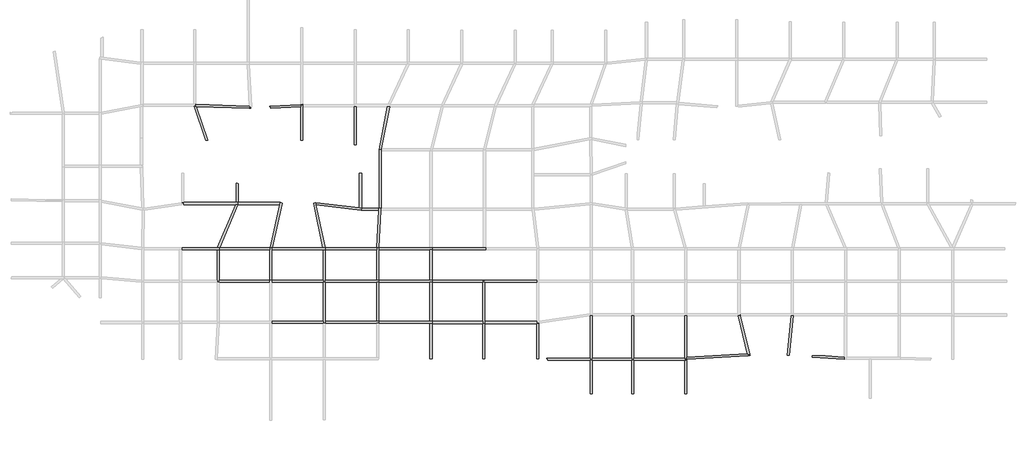
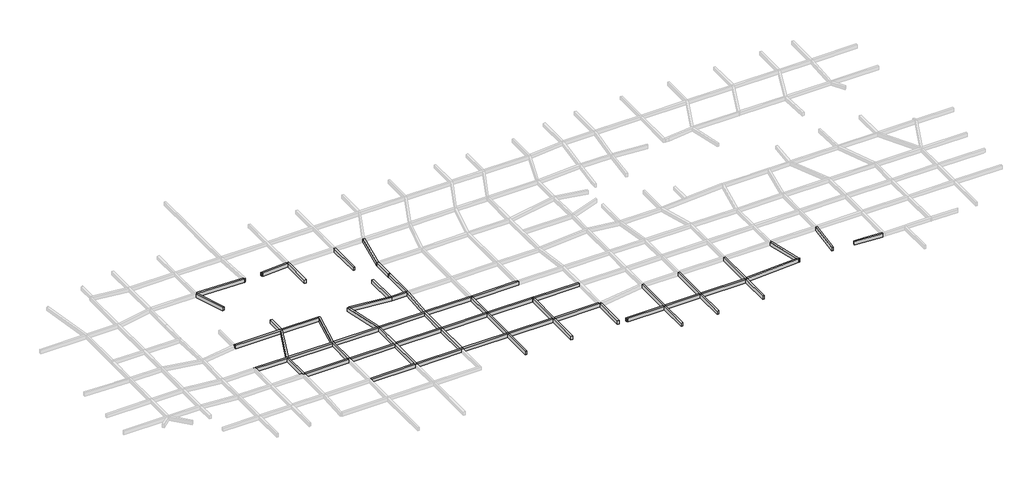
# One storey, part 4 of 15: 59 beams.
"""IFC4 building model written with IfcOpenShell, lengths in millimetres."""

from ifc_helpers import new_model, si_unit, frame, origin, place, context, project, spatial, polyline, outline, extrude, faceted_brep, element, save

model = new_model("IFC4")

# Units and contexts
model_context = context("Model", 3, world=origin())
ifc_project = project(units=[si_unit("LENGTHUNIT", "METRE", prefix="MILLI")], contexts=[model_context])

# Site, building, storey
site = spatial("IfcSite", under=ifc_project)
building = spatial("IfcBuilding", under=site)
storey = spatial("IfcBuildingStorey", under=building, Name="层高", Elevation=3300.0)

# Beams
placement = place(None, origin())
element("IfcBeam", 1, ObjectType="混凝土 - 矩形梁 : KL_beam", at=placement, inside=storey, context=model_context, shape_type="Brep", body=[
    faceted_brep([(169630.5037973, 63694.2273331, 3300.0), (169630.5037973, 63694.2273331, 2700.0), (169633.596084, 63790.1042703, 2700.0), (169633.596084, 63790.1042703, 3300.0), (169549.1301124, 63790.1042703, 2700.0), (169549.1301124, 63790.1042703, 3300.0), (169549.1301124, 63696.8518513, 2700.0), (169549.1301124, 63696.8518513, 3300.0)], [[[0, 1, 2, 3]], [[3, 2, 4, 5]], [[6, 7, 5, 4]], [[1, 0, 7, 6]], [[0, 3, 5, 7]], [[2, 1, 6, 4]]]),
    faceted_brep([(161497.8826169, 63956.5260367, 3300.0), (161497.8826169, 63956.5260367, 2700.0), (161712.9819644, 63949.5885096, 2700.0), (169429.1301124, 63700.722171, 2700.0), (169429.1301124, 63700.722171, 3300.0), (161712.9819644, 63949.5885096, 3300.0), (161650.300938, 63956.5260367, 3300.0), (161650.300938, 63956.5260367, 2700.0), (161650.300938, 64251.7661343, 3300.0), (161650.300938, 64251.7661343, 2700.0), (169429.1301124, 63790.1042703, 3300.0), (169429.1301124, 63910.1042703, 3300.0), (169481.9445066, 63910.1042703, 3300.0), (169477.2686164, 63999.3255706, 3300.0), (169477.2686164, 63999.3255706, 2700.0), (169481.9445066, 63910.1042703, 2700.0), (169429.1301124, 63910.1042703, 2700.0)], [[[0, 1, 2, 3, 4, 5]], [[6, 7, 1, 0]], [[7, 6, 8, 9]], [[6, 0, 5, 4, 10, 11, 12, 13, 8]], [[9, 8, 13, 14]], [[1, 7, 9, 14, 15, 16, 3, 2]], [[14, 13, 12, 15]], [[11, 16, 15, 12]], [[16, 11, 10, 4, 3]]]),
])
element("IfcBeam", 2, ObjectType="混凝土 - 矩形梁 : KL_beam", at=placement, inside=storey, context=model_context, shape_type="SweptSolid", body=[
    extrude(outline(polyline([(161393.3069779, 63956.5260367), (161497.8826169, 63956.5260367), (161712.9819644, 63949.5885096), (163398.0336281, 59055.8431382), (163080.7474238, 59055.8431382), (161393.3069779, 63956.5260367)])), frame((0.0, 0.0, 2700.0), z_axis=(0.0, 0.0, 1.0), x_axis=(1.0, 0.0, 0.0)), (0.0, 0.0, 1.0), 600.0),
])
element("IfcBeam", 3, ObjectType="混凝土 - 矩形梁 : KL_beam", at=placement, inside=storey, context=model_context, shape_type="Brep", body=[
    faceted_brep([(159257.4396146, 43339.5188273, 3300.0), (159549.7804968, 43339.3698411, 3300.0), (159549.7804968, 43042.2492414, 3300.0), (164749.7804968, 43042.2492414, 3300.0), (165049.7804968, 43042.2492414, 3300.0), (165049.7804968, 43342.2492414, 3300.0), (164801.5143118, 43342.2492414, 3300.0), (159257.5827095, 43342.2492414, 3300.0), (159549.7804968, 43042.2492414, 2700.0), (164749.7804968, 43042.2492414, 2700.0), (165049.7804968, 43042.2492414, 2700.0), (159549.7804968, 43339.3698411, 2700.0), (159257.4396146, 43339.5188273, 2700.0), (159257.5827095, 43342.2492414, 2700.0), (164801.5143118, 43342.2492414, 2700.0), (165049.7804968, 43342.2492414, 2700.0)], [[[0, 1, 2, 3, 4, 5, 6, 7]], [[2, 8, 9, 10, 4, 3]], [[11, 12, 13, 14, 15, 10, 9, 8]], [[5, 15, 14, 13, 7, 6]], [[11, 1, 0, 12]], [[1, 11, 8, 2]], [[5, 4, 10, 15]], [[7, 13, 12, 0]]]),
])
element("IfcBeam", 4, ObjectType="混凝土 - 矩形梁 : KL_beam", at=placement, inside=storey, context=model_context, shape_type="Brep", body=[
    faceted_brep([(164749.7804968, 38266.5295438, 3300.0), (165049.7804968, 38266.5295438, 3300.0), (165049.7804968, 38566.5295438, 3300.0), (165049.7804968, 43042.2492414, 3300.0), (164749.7804968, 43042.2492414, 3300.0), (164749.7804968, 38566.5295438, 3300.0), (164749.7804968, 38266.5295438, 2700.0), (164749.7804968, 43042.2492414, 2700.0), (164749.7804968, 38566.5295438, 2700.0), (165049.7804968, 38266.5295438, 2700.0), (165049.7804968, 43042.2492414, 2700.0), (165049.7804968, 38566.5295438, 2700.0)], [[[0, 1, 2, 3, 4, 5]], [[6, 0, 5, 4, 7, 8]], [[9, 6, 8, 7, 10, 11]], [[1, 9, 11, 10, 3, 2]], [[4, 3, 10, 7]], [[1, 0, 6, 9]]]),
])
element("IfcBeam", 5, ObjectType="混凝土 - 矩形梁 : KL_beam", at=placement, inside=storey, context=model_context, shape_type="SweptSolid", body=[
    extrude(outline(polyline([(165049.7804968, 38266.5295438), (165049.7804968, 38566.5295438), (172449.7804968, 38566.5295438), (172449.7804968, 38266.5295438), (165049.7804968, 38266.5295438)])), frame((0.0, 0.0, 2700.0), z_axis=(0.0, 0.0, 1.0), x_axis=(1.0, 0.0, 0.0)), (0.0, 0.0, 1.0), 600.0),
])
element("IfcBeam", 6, ObjectType="混凝土 - 矩形梁 : KL_beam", at=placement, inside=storey, context=model_context, shape_type="Brep", body=[
    faceted_brep([(172749.7804968, 43342.2492414, 3300.0), (172481.1122271, 43342.2492414, 3300.0), (172449.7804968, 43342.2492414, 3300.0), (172449.7804968, 43042.2492414, 3300.0), (172449.7804968, 38566.5295438, 3300.0), (172749.7804968, 38566.5295438, 3300.0), (172749.7804968, 43042.2492414, 3300.0), (172449.7804968, 43342.2492414, 2700.0), (172449.7804968, 43042.2492414, 2700.0), (172449.7804968, 38566.5295438, 2700.0), (172481.1122271, 43342.2492414, 2700.0), (172749.7804968, 43342.2492414, 2700.0), (172749.7804968, 43042.2492414, 2700.0), (172749.7804968, 38566.5295438, 2700.0)], [[[0, 1, 2, 3, 4, 5, 6]], [[2, 7, 8, 9, 4, 3]], [[7, 10, 11, 12, 13, 9, 8]], [[11, 0, 6, 5, 13, 12]], [[5, 4, 9, 13]], [[2, 1, 0, 11, 10, 7]]]),
])
element("IfcBeam", 7, ObjectType="混凝土 - 矩形梁 : KL_beam", at=placement, inside=storey, context=model_context, shape_type="Brep", body=[
    faceted_brep([(165049.7804968, 43342.2492414, 3300.0), (165049.7804968, 43042.2492414, 3300.0), (172449.7804968, 43042.2492414, 3300.0), (172449.7804968, 43342.2492414, 3300.0), (165127.2075965, 43342.2492414, 3300.0), (165049.7804968, 43042.2492414, 2700.0), (172449.7804968, 43042.2492414, 2700.0), (165049.7804968, 43342.2492414, 2700.0), (165127.2075965, 43342.2492414, 2700.0), (172449.7804968, 43342.2492414, 2700.0)], [[[0, 1, 2, 3, 4]], [[1, 5, 6, 2]], [[5, 7, 8, 9, 6]], [[7, 0, 4, 3, 9, 8]], [[1, 0, 7, 5]], [[3, 2, 6, 9]]]),
])
element("IfcBeam", 8, ObjectType="混凝土 - 矩形梁 : KL_beam", at=placement, inside=storey, context=model_context, shape_type="Brep", body=[
    faceted_brep([(180549.7804968, 43042.2492414, 3300.0), (180549.7804968, 43342.2492414, 3300.0), (180520.652311, 43342.2492414, 3300.0), (180213.9501326, 43342.2492414, 3300.0), (172789.0034594, 43342.2492414, 3300.0), (172749.7804968, 43342.2492414, 3300.0), (172749.7804968, 43042.2492414, 3300.0), (180249.7804968, 43042.2492414, 3300.0), (180549.7804968, 43042.2492414, 2700.0), (172749.7804968, 43042.2492414, 2700.0), (180249.7804968, 43042.2492414, 2700.0), (180549.7804968, 43342.2492414, 2700.0), (172749.7804968, 43342.2492414, 2700.0), (172789.0034594, 43342.2492414, 2700.0), (180213.9501326, 43342.2492414, 2700.0), (180520.652311, 43342.2492414, 2700.0)], [[[0, 1, 2, 3, 4, 5, 6, 7]], [[8, 0, 7, 6, 9, 10]], [[11, 8, 10, 9, 12, 13, 14, 15]], [[1, 11, 15, 14, 13, 12, 5, 4, 3, 2]], [[6, 5, 12, 9]], [[1, 0, 8, 11]]]),
])
element("IfcBeam", 9, ObjectType="混凝土 - 矩形梁 : KL_beam", at=placement, inside=storey, context=model_context, shape_type="Brep", body=[
    faceted_brep([(180249.7804968, 38266.5295438, 3300.0), (180549.7804968, 38266.5295438, 3300.0), (180549.7804968, 38566.5295438, 3300.0), (180549.7804968, 43042.2492414, 3300.0), (180249.7804968, 43042.2492414, 3300.0), (180249.7804968, 38566.5295438, 3300.0), (180549.7804968, 38266.5295438, 2700.0), (180549.7804968, 38566.5295438, 2700.0), (180549.7804968, 43042.2492414, 2700.0), (180249.7804968, 38266.5295438, 2700.0), (180249.7804968, 38566.5295438, 2700.0), (180249.7804968, 43042.2492414, 2700.0)], [[[0, 1, 2, 3, 4, 5]], [[1, 6, 7, 8, 3, 2]], [[6, 9, 10, 11, 8, 7]], [[9, 0, 5, 4, 11, 10]], [[4, 3, 8, 11]], [[1, 0, 9, 6]]]),
])
element("IfcBeam", 10, ObjectType="混凝土 - 矩形梁 : KL_beam", at=placement, inside=storey, context=model_context, shape_type="SweptSolid", body=[
    extrude(outline(polyline([(172749.7804968, 38266.5295438), (172749.7804968, 38566.5295438), (180249.7804968, 38566.5295438), (180249.7804968, 38266.5295438), (172749.7804968, 38266.5295438)])), frame((0.0, 0.0, 2700.0), z_axis=(0.0, 0.0, 1.0), x_axis=(1.0, 0.0, 0.0)), (0.0, 0.0, 1.0), 600.0),
])
element("IfcBeam", 11, ObjectType="混凝土 - 矩形梁 : KL_beam", at=placement, inside=storey, context=model_context, shape_type="Brep", body=[
    faceted_brep([(180249.7804968, 32266.5295438, 3300.0), (180549.7804968, 32266.5295438, 3300.0), (180549.7804968, 32566.5295438, 3300.0), (180549.7804968, 38266.5295438, 3300.0), (180249.7804968, 38266.5295438, 3300.0), (180249.7804968, 32566.5295438, 3300.0), (180249.7804968, 32266.5295438, 2700.0), (180249.7804968, 38266.5295438, 2700.0), (180249.7804968, 32566.5295438, 2700.0), (180549.7804968, 32266.5295438, 2700.0), (180549.7804968, 38266.5295438, 2700.0), (180549.7804968, 32566.5295438, 2700.0)], [[[0, 1, 2, 3, 4, 5]], [[6, 0, 5, 4, 7, 8]], [[9, 6, 8, 7, 10, 11]], [[1, 9, 11, 10, 3, 2]], [[4, 3, 10, 7]], [[1, 0, 6, 9]]]),
])
element("IfcBeam", 12, ObjectType="混凝土 - 矩形梁 : KL_beam", at=placement, inside=storey, context=model_context, shape_type="SweptSolid", body=[
    extrude(outline(polyline([(172749.7804968, 32266.5295438), (172749.7804968, 32566.5295438), (180249.7804968, 32566.5295438), (180249.7804968, 32266.5295438), (172749.7804968, 32266.5295438)])), frame((0.0, 0.0, 2700.0), z_axis=(0.0, 0.0, 1.0), x_axis=(1.0, 0.0, 0.0)), (0.0, 0.0, 1.0), 600.0),
])
element("IfcBeam", 13, ObjectType="混凝土 - 矩形梁 : KL_beam", at=placement, inside=storey, context=model_context, shape_type="Brep", body=[
    faceted_brep([(188349.7804968, 32266.5295438, 3300.0), (188349.7804968, 32566.5295438, 3300.0), (188049.7804968, 32566.5295438, 3300.0), (180549.7804968, 32566.5295438, 3300.0), (180549.7804968, 32266.5295438, 3300.0), (188049.7804968, 32266.5295438, 3300.0), (188349.7804968, 32266.5295438, 2700.0), (180549.7804968, 32266.5295438, 2700.0), (188049.7804968, 32266.5295438, 2700.0), (188349.7804968, 32566.5295438, 2700.0), (180549.7804968, 32566.5295438, 2700.0), (188049.7804968, 32566.5295438, 2700.0)], [[[0, 1, 2, 3, 4, 5]], [[6, 0, 5, 4, 7, 8]], [[9, 6, 8, 7, 10, 11]], [[1, 9, 11, 10, 3, 2]], [[4, 3, 10, 7]], [[1, 0, 6, 9]]]),
])
element("IfcBeam", 14, ObjectType="混凝土 - 矩形梁 : KL_beam", at=placement, inside=storey, context=model_context, shape_type="Brep", body=[
    faceted_brep([(188349.7804968, 38266.5295438, 3300.0), (188349.7804968, 38566.5295438, 3300.0), (188049.7804968, 38566.5295438, 3300.0), (180549.7804968, 38566.5295438, 3300.0), (180549.7804968, 38266.5295438, 3300.0), (188049.7804968, 38266.5295438, 3300.0), (188349.7804968, 38266.5295438, 2700.0), (180549.7804968, 38266.5295438, 2700.0), (188049.7804968, 38266.5295438, 2700.0), (188349.7804968, 38566.5295438, 2700.0), (180549.7804968, 38566.5295438, 2700.0), (188049.7804968, 38566.5295438, 2700.0)], [[[0, 1, 2, 3, 4, 5]], [[6, 0, 5, 4, 7, 8]], [[9, 6, 8, 7, 10, 11]], [[1, 9, 11, 10, 3, 2]], [[4, 3, 10, 7]], [[1, 0, 6, 9]]]),
])
element("IfcBeam", 15, ObjectType="混凝土 - 矩形梁 : KL_beam", at=placement, inside=storey, context=model_context, shape_type="SweptSolid", body=[
    extrude(outline(polyline([(188349.7804968, 32566.5295438), (188049.7804968, 32566.5295438), (188049.7804968, 38266.5295438), (188349.7804968, 38266.5295438), (188349.7804968, 32566.5295438)])), frame((0.0, 0.0, 2700.0), z_axis=(0.0, 0.0, 1.0), x_axis=(1.0, 0.0, 0.0)), (0.0, 0.0, 1.0), 600.0),
])
element("IfcBeam", 16, ObjectType="混凝土 - 矩形梁 : KL_beam", at=placement, inside=storey, context=model_context, shape_type="Brep", body=[
    faceted_brep([(188349.7804968, 43342.2492414, 3300.0), (188057.5827095, 43342.2492414, 3300.0), (188049.7804968, 43342.2492414, 3300.0), (188049.7804968, 43042.2492414, 3300.0), (188049.7804968, 38566.5295438, 3300.0), (188349.7804968, 38566.5295438, 3300.0), (188349.7804968, 43042.2492414, 3300.0), (188049.7804968, 43342.2492414, 2700.0), (188049.7804968, 43042.2492414, 2700.0), (188049.7804968, 38566.5295438, 2700.0), (188057.5827095, 43342.2492414, 2700.0), (188349.7804968, 43342.2492414, 2700.0), (188349.7804968, 43042.2492414, 2700.0), (188349.7804968, 38566.5295438, 2700.0)], [[[0, 1, 2, 3, 4, 5, 6]], [[2, 7, 8, 9, 4, 3]], [[7, 10, 11, 12, 13, 9, 8]], [[11, 0, 6, 5, 13, 12]], [[5, 4, 9, 13]], [[2, 1, 0, 11, 10, 7]]]),
])
element("IfcBeam", 17, ObjectType="混凝土 - 矩形梁 : KL_beam", at=placement, inside=storey, context=model_context, shape_type="SweptSolid", body=[
    extrude(outline(polyline([(180549.7804968, 43042.2492414), (180549.7804968, 43342.2492414), (188049.7804968, 43342.2492414), (188049.7804968, 43042.2492414), (180549.7804968, 43042.2492414)])), frame((0.0, 0.0, 2700.0), z_axis=(0.0, 0.0, 1.0), x_axis=(1.0, 0.0, 0.0)), (0.0, 0.0, 1.0), 600.0),
])
element("IfcBeam", 18, ObjectType="混凝土 - 矩形梁 : KL_beam", at=placement, inside=storey, context=model_context, shape_type="Brep", body=[
    faceted_brep([(196149.7804968, 43042.2492414, 3300.0), (196149.7804968, 43342.2492414, 3300.0), (195849.7804968, 43342.2492414, 3300.0), (188357.9944133, 43342.2492414, 3300.0), (188349.7804968, 43342.2492414, 3300.0), (188349.7804968, 43042.2492414, 3300.0), (195849.7804968, 43042.2492414, 3300.0), (196149.7804968, 43042.2492414, 2700.0), (188349.7804968, 43042.2492414, 2700.0), (195849.7804968, 43042.2492414, 2700.0), (196149.7804968, 43342.2492414, 2700.0), (188349.7804968, 43342.2492414, 2700.0), (188357.9944133, 43342.2492414, 2700.0), (195849.7804968, 43342.2492414, 2700.0)], [[[0, 1, 2, 3, 4, 5, 6]], [[7, 0, 6, 5, 8, 9]], [[10, 7, 9, 8, 11, 12, 13]], [[1, 10, 13, 12, 11, 4, 3, 2]], [[5, 4, 11, 8]], [[1, 0, 7, 10]]]),
])
element("IfcBeam", 19, ObjectType="混凝土 - 矩形梁 : KL_beam", at=placement, inside=storey, context=model_context, shape_type="Brep", body=[
    faceted_brep([(196149.7804968, 38266.5295438, 3300.0), (196149.7804968, 38566.5295438, 3300.0), (195849.7804968, 38566.5295438, 3300.0), (188349.7804968, 38566.5295438, 3300.0), (188349.7804968, 38266.5295438, 3300.0), (195849.7804968, 38266.5295438, 3300.0), (196149.7804968, 38266.5295438, 2700.0), (188349.7804968, 38266.5295438, 2700.0), (195849.7804968, 38266.5295438, 2700.0), (196149.7804968, 38566.5295438, 2700.0), (188349.7804968, 38566.5295438, 2700.0), (195849.7804968, 38566.5295438, 2700.0)], [[[0, 1, 2, 3, 4, 5]], [[6, 0, 5, 4, 7, 8]], [[9, 6, 8, 7, 10, 11]], [[1, 9, 11, 10, 3, 2]], [[4, 3, 10, 7]], [[1, 0, 6, 9]]]),
])
element("IfcBeam", 20, ObjectType="混凝土 - 矩形梁 : KL_beam", at=placement, inside=storey, context=model_context, shape_type="Brep", body=[
    faceted_brep([(196149.7804968, 32266.5295438, 3300.0), (196149.7804968, 32542.26105, 3300.0), (196149.7804968, 32566.5295438, 3300.0), (195849.7804968, 32566.5295438, 3300.0), (188349.7804968, 32566.5295438, 3300.0), (188349.7804968, 32266.5295438, 3300.0), (195849.7804968, 32266.5295438, 3300.0), (196149.7804968, 32266.5295438, 2700.0), (188349.7804968, 32266.5295438, 2700.0), (195849.7804968, 32266.5295438, 2700.0), (196149.7804968, 32566.5295438, 2700.0), (196149.7804968, 32542.26105, 2700.0), (188349.7804968, 32566.5295438, 2700.0), (195849.7804968, 32566.5295438, 2700.0)], [[[0, 1, 2, 3, 4, 5, 6]], [[7, 0, 6, 5, 8, 9]], [[10, 11, 7, 9, 8, 12, 13]], [[2, 10, 13, 12, 4, 3]], [[5, 4, 12, 8]], [[2, 1, 0, 7, 11, 10]]]),
])
element("IfcBeam", 21, ObjectType="混凝土 - 矩形梁 : KL_beam", at=placement, inside=storey, context=model_context, shape_type="SweptSolid", body=[
    extrude(outline(polyline([(195849.7804968, 38266.5295438), (196149.7804968, 38266.5295438), (196149.7804968, 32566.5295438), (195849.7804968, 32566.5295438), (195849.7804968, 38266.5295438)])), frame((0.0, 0.0, 2700.0), z_axis=(0.0, 0.0, 1.0), x_axis=(1.0, 0.0, 0.0)), (0.0, 0.0, 1.0), 600.0),
])
element("IfcBeam", 22, ObjectType="混凝土 - 矩形梁 : KL_beam", at=placement, inside=storey, context=model_context, shape_type="SweptSolid", body=[
    extrude(outline(polyline([(195849.7804968, 43042.2492414), (196149.7804968, 43042.2492414), (196149.7804968, 38566.5295438), (195849.7804968, 38566.5295438), (195849.7804968, 43042.2492414)])), frame((0.0, 0.0, 2700.0), z_axis=(0.0, 0.0, 1.0), x_axis=(1.0, 0.0, 0.0)), (0.0, 0.0, 1.0), 600.0),
])
element("IfcBeam", 23, ObjectType="混凝土 - 矩形梁 : KL_beam", at=placement, inside=storey, context=model_context, shape_type="Brep", body=[
    faceted_brep([(174002.1069516, 49930.4011957, 3300.0), (173932.8464943, 49630.4011957, 3300.0), (172481.1122271, 43342.2492414, 3300.0), (172749.7804968, 43342.2492414, 3300.0), (172789.0034594, 43342.2492414, 3300.0), (174275.6873874, 49781.7848082, 3300.0), (174260.3009401, 49781.7848082, 3300.0), (174140.3009401, 49781.7848082, 3300.0), (174140.3009401, 49898.4965996, 3300.0), (172789.0034594, 43342.2492414, 2700.0), (174275.6873874, 49781.7848082, 2700.0), (172481.1122271, 43342.2492414, 2700.0), (173932.8464943, 49630.4011957, 2700.0), (174002.1069516, 49930.4011957, 2700.0), (174140.3009401, 49898.4965996, 2700.0), (174140.3009401, 49781.7848082, 2700.0), (172749.7804968, 43342.2492414, 2700.0)], [[[0, 1, 2, 3, 4, 5, 6, 7, 8]], [[4, 9, 10, 5]], [[11, 12, 13, 14, 15, 10, 9, 16]], [[2, 1, 0, 13, 12, 11]], [[2, 11, 16, 9, 4, 3]], [[13, 0, 8, 14]], [[7, 15, 14, 8]], [[15, 7, 6, 5, 10]]]),
])
element("IfcBeam", 24, ObjectType="混凝土 - 矩形梁 : KL_beam", at=placement, inside=storey, context=model_context, shape_type="Brep", body=[
    faceted_brep([(180520.652311, 43342.2492414, 3300.0), (179195.182726, 49578.0933603, 3300.0), (179129.3076558, 49888.0111993, 3300.0), (179060.3009401, 49873.3433691, 3300.0), (179060.3009401, 49781.7848082, 3300.0), (178845.1845937, 49781.7848082, 3300.0), (180213.9501326, 43342.2492414, 3300.0), (180249.7804968, 43342.2492414, 3300.0), (180520.652311, 43342.2492414, 2700.0), (179195.182726, 49578.0933603, 2700.0), (179129.3076558, 49888.0111993, 2700.0), (180249.7804968, 43342.2492414, 2700.0), (180213.9501326, 43342.2492414, 2700.0), (178845.1845937, 49781.7848082, 2700.0), (179060.3009401, 49781.7848082, 2700.0), (179060.3009401, 49873.3433691, 2700.0)], [[[0, 1, 2, 3, 4, 5, 6, 7]], [[2, 1, 0, 8, 9, 10]], [[10, 9, 8, 11, 12, 13, 14, 15]], [[12, 6, 5, 13]], [[8, 0, 7, 6, 12, 11]], [[2, 10, 15, 3]], [[4, 14, 13, 5]], [[14, 4, 3, 15]]]),
])
element("IfcBeam", 25, ObjectType="混凝土 - 矩形梁 : KL_beam", at=placement, inside=storey, context=model_context, shape_type="Brep", body=[
    faceted_brep([(167784.8242353, 49930.4011957, 3300.0), (167535.3734044, 49930.4011957, 3300.0), (159895.197808, 49930.4011957, 3300.0), (159602.853123, 49930.4011957, 3300.0), (159601.8562875, 49911.380442, 3300.0), (159901.445148, 49895.6796551, 3300.0), (159888.5393285, 49649.4219495, 3300.0), (159887.542493, 49630.4011957, 3300.0), (167459.1309506, 49630.4011957, 3300.0), (167784.8242353, 49630.4011957, 3300.0), (159887.542493, 49630.4011957, 2700.0), (167459.1309506, 49630.4011957, 2700.0), (167784.8242353, 49630.4011957, 2700.0), (159602.853123, 49930.4011957, 2700.0), (159895.197808, 49930.4011957, 2700.0), (167535.3734044, 49930.4011957, 2700.0), (167784.8242353, 49930.4011957, 2700.0), (159888.5393285, 49649.4219495, 2700.0), (159901.445148, 49895.6796551, 2700.0), (159601.8562875, 49911.380442, 2700.0)], [[[0, 1, 2, 3, 4, 5, 6, 7, 8, 9]], [[9, 8, 7, 10, 11, 12]], [[13, 14, 15, 16, 12, 11, 10, 17, 18, 19]], [[3, 2, 1, 0, 16, 15, 14, 13]], [[19, 4, 3, 13]], [[5, 18, 17, 10, 7, 6]], [[18, 5, 4, 19]], [[0, 9, 12, 16]]]),
])
element("IfcBeam", 26, ObjectType="混凝土 - 矩形梁 : KL_beam", at=placement, inside=storey, context=model_context, shape_type="Brep", body=[
    faceted_brep([(173932.8464943, 49630.4011957, 3300.0), (174002.1069516, 49930.4011957, 3300.0), (167835.3734044, 49930.4011957, 3300.0), (167784.8242353, 49930.4011957, 3300.0), (167784.8242353, 49630.4011957, 3300.0), (173932.8464943, 49630.4011957, 2700.0), (167784.8242353, 49630.4011957, 2700.0), (174002.1069516, 49930.4011957, 2700.0), (167784.8242353, 49930.4011957, 2700.0), (167835.3734044, 49930.4011957, 2700.0)], [[[0, 1, 2, 3, 4]], [[5, 0, 4, 6]], [[7, 5, 6, 8, 9]], [[1, 7, 9, 8, 3, 2]], [[1, 0, 5, 7]], [[4, 3, 8, 6]]]),
])
element("IfcBeam", 27, ObjectType="混凝土 - 矩形梁 : KL_beam", at=placement, inside=storey, context=model_context, shape_type="Brep", body=[
    faceted_brep([(165127.2075965, 43342.2492414, 3300.0), (167784.8242353, 49630.4011957, 3300.0), (167459.1309506, 49630.4011957, 3300.0), (164801.5143118, 43342.2492414, 3300.0), (165049.7804968, 43342.2492414, 3300.0), (164801.5143118, 43342.2492414, 2700.0), (167459.1309506, 49630.4011957, 2700.0), (167784.8242353, 49630.4011957, 2700.0), (165127.2075965, 43342.2492414, 2700.0), (165049.7804968, 43342.2492414, 2700.0)], [[[0, 1, 2, 3, 4]], [[5, 3, 2, 6]], [[7, 8, 9, 5, 6]], [[1, 0, 8, 7]], [[3, 5, 9, 8, 0, 4]], [[2, 1, 7, 6]]]),
])
element("IfcBeam", 28, ObjectType="混凝土 - 矩形梁 : KL_beam", at=placement, inside=storey, context=model_context, shape_type="Brep", body=[
    faceted_brep([(167535.3734044, 52741.7848082, 2700.0), (167535.3734044, 52741.7848082, 3300.0), (167685.197808, 52741.7848082, 3300.0), (167685.197808, 52741.7848082, 2700.0), (167535.3734044, 49930.4011957, 3300.0), (167784.8242353, 49930.4011957, 3300.0), (167835.3734044, 49930.4011957, 3300.0), (167835.3734044, 52681.7848082, 3300.0), (167805.197808, 52681.7848082, 3300.0), (167685.197808, 52681.7848082, 3300.0), (167835.3734044, 49930.4011957, 2700.0), (167835.3734044, 52681.7848082, 2700.0), (167535.3734044, 49930.4011957, 2700.0), (167685.197808, 52681.7848082, 2700.0), (167784.8242353, 49930.4011957, 2700.0)], [[[0, 1, 2, 3]], [[1, 4, 5, 6, 7, 8, 9, 2]], [[6, 10, 11, 7]], [[12, 0, 3, 13, 11, 10, 14]], [[1, 0, 12, 4]], [[4, 12, 14, 10, 6, 5]], [[9, 13, 3, 2]], [[13, 9, 8, 7, 11]]]),
])
element("IfcBeam", 29, ObjectType="混凝土 - 矩形梁 : KL_beam", at=placement, inside=storey, context=model_context, shape_type="Brep", body=[
    faceted_brep([(188057.5827095, 43342.2492414, 3300.0), (188349.7804968, 43342.2492414, 3300.0), (188357.9944133, 43342.2492414, 3300.0), (188644.4147836, 48807.4754781, 3300.0), (188660.1371174, 49107.4754781, 3300.0), (188410.3816443, 49107.4754781, 3300.0), (188359.7254136, 49107.4754781, 3300.0), (188344.0030798, 48807.4754781, 3300.0), (188660.1371174, 49107.4754781, 2700.0), (188357.9944133, 43342.2492414, 2700.0), (188644.4147836, 48807.4754781, 2700.0), (188349.7804968, 43342.2492414, 2700.0), (188057.5827095, 43342.2492414, 2700.0), (188344.0030798, 48807.4754781, 2700.0), (188359.7254136, 49107.4754781, 2700.0), (188410.3816443, 49107.4754781, 2700.0)], [[[0, 1, 2, 3, 4, 5, 6, 7]], [[8, 4, 3, 2, 9, 10]], [[9, 11, 12, 13, 14, 15, 8, 10]], [[12, 0, 7, 6, 14, 13]], [[0, 12, 11, 9, 2, 1]], [[6, 5, 4, 8, 15, 14]]]),
])
element("IfcBeam", 30, ObjectType="混凝土 - 矩形梁 : KL_beam", at=placement, inside=storey, context=model_context, shape_type="Brep", body=[
    faceted_brep([(203965.7079926, 43042.2492414, 3300.0), (203965.7079926, 43342.2492414, 3300.0), (203665.7079926, 43342.2492414, 3300.0), (196149.7804968, 43342.2492414, 3300.0), (196149.7804968, 43042.2492414, 3300.0), (203965.7079926, 43042.2492414, 2700.0), (196149.7804968, 43042.2492414, 2700.0), (203965.7079926, 43342.2492414, 2700.0), (196149.7804968, 43342.2492414, 2700.0), (203665.7079926, 43342.2492414, 2700.0)], [[[0, 1, 2, 3, 4]], [[5, 0, 4, 6]], [[7, 5, 6, 8, 9]], [[1, 7, 9, 8, 3, 2]], [[4, 3, 8, 6]], [[1, 0, 5, 7]]]),
])
element("IfcBeam", 31, ObjectType="混凝土 - 矩形梁 : KL_beam", at=placement, inside=storey, context=model_context, shape_type="Brep", body=[
    faceted_brep([(203565.7078837, 38542.26105, 3300.0), (203565.7078837, 38266.5295438, 3300.0), (203565.7078837, 38242.26105, 3300.0), (203865.7078837, 38242.26105, 3300.0), (211449.7804968, 38242.26105, 3300.0), (211449.7804968, 38542.26105, 3300.0), (203865.7078837, 38542.26105, 3300.0), (203565.7078837, 38542.26105, 2700.0), (211449.7804968, 38542.26105, 2700.0), (203865.7078837, 38542.26105, 2700.0), (203565.7078837, 38242.26105, 2700.0), (203565.7078837, 38266.5295438, 2700.0), (211449.7804968, 38242.26105, 2700.0), (203865.7078837, 38242.26105, 2700.0)], [[[0, 1, 2, 3, 4, 5, 6]], [[7, 0, 6, 5, 8, 9]], [[10, 11, 7, 9, 8, 12, 13]], [[2, 10, 13, 12, 4, 3]], [[5, 4, 12, 8]], [[2, 1, 0, 7, 11, 10]]]),
])
element("IfcBeam", 32, ObjectType="混凝土 - 矩形梁 : KL_beam", at=placement, inside=storey, context=model_context, shape_type="Brep", body=[
    faceted_brep([(203565.7078837, 32242.26105, 3300.0), (203865.7078837, 32242.26105, 3300.0), (203865.7078837, 32542.26105, 3300.0), (203865.7078837, 38242.26105, 3300.0), (203565.7078837, 38242.26105, 3300.0), (203565.7078837, 32542.26105, 3300.0), (203565.7078837, 32242.26105, 2700.0), (203565.7078837, 38242.26105, 2700.0), (203565.7078837, 32542.26105, 2700.0), (203865.7078837, 32242.26105, 2700.0), (203865.7078837, 38242.26105, 2700.0), (203865.7078837, 32542.26105, 2700.0)], [[[0, 1, 2, 3, 4, 5]], [[6, 0, 5, 4, 7, 8]], [[9, 6, 8, 7, 10, 11]], [[1, 9, 11, 10, 3, 2]], [[4, 3, 10, 7]], [[1, 0, 6, 9]]]),
])
element("IfcBeam", 33, ObjectType="混凝土 - 矩形梁 : KL_beam", at=placement, inside=storey, context=model_context, shape_type="Brep", body=[
    faceted_brep([(195849.7804968, 32266.5295438, 3300.0), (195849.7804968, 32242.26105, 3300.0), (196149.7804968, 32242.26105, 3300.0), (203565.7078837, 32242.26105, 3300.0), (203565.7078837, 32542.26105, 3300.0), (196149.7804968, 32542.26105, 3300.0), (196149.7804968, 32266.5295438, 3300.0), (196149.7804968, 32542.26105, 2700.0), (203565.7078837, 32542.26105, 2700.0), (195849.7804968, 32242.26105, 2700.0), (195849.7804968, 32266.5295438, 2700.0), (196149.7804968, 32266.5295438, 2700.0), (203565.7078837, 32242.26105, 2700.0), (196149.7804968, 32242.26105, 2700.0)], [[[0, 1, 2, 3, 4, 5, 6]], [[7, 5, 4, 8]], [[9, 10, 11, 7, 8, 12, 13]], [[1, 9, 13, 12, 3, 2]], [[9, 1, 0, 10]], [[6, 11, 10, 0]], [[11, 6, 5, 7]], [[4, 3, 12, 8]]]),
])
element("IfcBeam", 34, ObjectType="混凝土 - 矩形梁 : KL_beam", at=placement, inside=storey, context=model_context, shape_type="SweptSolid", body=[
    extrude(outline(polyline([(196149.7804968, 38566.5295438), (203865.7078837, 38566.5295438), (203865.7078837, 38542.26105), (203565.7078837, 38542.26105), (203565.7078837, 38266.5295438), (196149.7804968, 38266.5295438), (196149.7804968, 38566.5295438)])), frame((0.0, 0.0, 2700.0), z_axis=(0.0, 0.0, 1.0), x_axis=(1.0, 0.0, 0.0)), (0.0, 0.0, 1.0), 600.0),
])
element("IfcBeam", 35, ObjectType="混凝土 - 矩形梁 : KL_beam", at=placement, inside=storey, context=model_context, shape_type="Brep", body=[
    faceted_brep([(203865.7078837, 32242.26105, 3300.0), (211449.7804968, 32242.26105, 3300.0), (211749.7804968, 32242.26105, 3300.0), (211749.7804968, 32262.7548984, 3300.0), (211449.7804968, 32262.7548984, 3300.0), (211449.7804968, 32521.7672016, 3300.0), (211449.7804968, 32542.26105, 3300.0), (203865.7078837, 32542.26105, 3300.0), (203865.7078837, 32542.26105, 2700.0), (211449.7804968, 32542.26105, 2700.0), (211749.7804968, 32242.26105, 2700.0), (211449.7804968, 32242.26105, 2700.0), (203865.7078837, 32242.26105, 2700.0), (211449.7804968, 32521.7672016, 2700.0), (211449.7804968, 32262.7548984, 2700.0), (211749.7804968, 32262.7548984, 2700.0)], [[[0, 1, 2, 3, 4, 5, 6, 7]], [[8, 7, 6, 9]], [[10, 11, 12, 8, 9, 13, 14, 15]], [[2, 1, 0, 12, 11, 10]], [[15, 3, 2, 10]], [[0, 7, 8, 12]], [[4, 14, 13, 9, 6, 5]], [[14, 4, 3, 15]]]),
])
element("IfcBeam", 36, ObjectType="混凝土 - 矩形梁 : KL_beam", at=placement, inside=storey, context=model_context, shape_type="SweptSolid", body=[
    extrude(outline(polyline([(211449.7804968, 32242.26105), (211749.7804968, 32242.26105), (211749.7804968, 27102.1039685), (211449.7804968, 27102.1039685), (211449.7804968, 32242.26105)])), frame((0.0, 0.0, 2700.0), z_axis=(0.0, 0.0, 1.0), x_axis=(1.0, 0.0, 0.0)), (0.0, 0.0, 1.0), 600.0),
])
element("IfcBeam", 37, ObjectType="混凝土 - 矩形梁 : KL_beam", at=placement, inside=storey, context=model_context, shape_type="Brep", body=[
    faceted_brep([(219549.7804968, 33412.7548984, 3300.0), (219249.7804968, 33368.5241292, 3300.0), (219249.7804968, 27192.1039685, 3300.0), (219249.7804968, 26892.1039685, 3300.0), (219549.7804968, 26892.1039685, 3300.0), (219549.7804968, 27192.1039685, 3300.0), (219549.7804968, 33392.26105, 3300.0), (219249.7804968, 33368.5241292, 2700.0), (219249.7804968, 27192.1039685, 2700.0), (219249.7804968, 26892.1039685, 2700.0), (219549.7804968, 33412.7548984, 2700.0), (219549.7804968, 33392.26105, 2700.0), (219549.7804968, 27192.1039685, 2700.0), (219549.7804968, 26892.1039685, 2700.0)], [[[0, 1, 2, 3, 4, 5, 6]], [[1, 7, 8, 9, 3, 2]], [[7, 10, 11, 12, 13, 9, 8]], [[10, 0, 6, 5, 4, 13, 12, 11]], [[1, 0, 10, 7]], [[4, 3, 9, 13]]]),
])
element("IfcBeam", 38, ObjectType="混凝土 - 矩形梁 : KL_beam", at=placement, inside=storey, context=model_context, shape_type="Brep", body=[
    faceted_brep([(225349.7804968, 26892.1039685, 3300.0), (225649.7804968, 26892.1039685, 3300.0), (225649.7804968, 27192.1039685, 3300.0), (225649.7804968, 33392.26105, 3300.0), (225349.7804968, 33392.26105, 3300.0), (225349.7804968, 27192.1039685, 3300.0), (225349.7804968, 26892.1039685, 2700.0), (225349.7804968, 33392.26105, 2700.0), (225349.7804968, 27192.1039685, 2700.0), (225649.7804968, 26892.1039685, 2700.0), (225649.7804968, 33392.26105, 2700.0), (225649.7804968, 27192.1039685, 2700.0)], [[[0, 1, 2, 3, 4, 5]], [[6, 0, 5, 4, 7, 8]], [[9, 6, 8, 7, 10, 11]], [[1, 9, 11, 10, 3, 2]], [[4, 3, 10, 7]], [[1, 0, 6, 9]]]),
])
element("IfcBeam", 39, ObjectType="混凝土 - 矩形梁 : KL_beam", at=placement, inside=storey, context=model_context, shape_type="Brep", body=[
    faceted_brep([(233049.8189959, 27001.348591, 3300.0), (233349.8189959, 27001.348591, 3300.0), (233349.8189959, 27301.9346528, 3300.0), (233349.8189959, 33392.26105, 3300.0), (233049.8189959, 33392.26105, 3300.0), (233049.8189959, 27192.1039685, 3300.0), (233049.8189959, 27001.348591, 2700.0), (233049.8189959, 33392.26105, 2700.0), (233049.8189959, 27192.1039685, 2700.0), (233349.8189959, 27001.348591, 2700.0), (233349.8189959, 33392.26105, 2700.0), (233349.8189959, 27301.9346528, 2700.0)], [[[0, 1, 2, 3, 4, 5]], [[6, 0, 5, 4, 7, 8]], [[9, 6, 8, 7, 10, 11]], [[1, 9, 11, 10, 3, 2]], [[4, 3, 10, 7]], [[1, 0, 6, 9]]]),
])
element("IfcBeam", 40, ObjectType="混凝土 - 矩形梁 : KL_beam", at=placement, inside=storey, context=model_context, shape_type="Brep", body=[
    faceted_brep([(242283.1006534, 27662.5311529, 3300.0), (242362.2332925, 27660.5871631, 3300.0), (242365.1803497, 27780.5509696, 3300.0), (242564.2767952, 27775.6599226, 3300.0), (241190.9158106, 33392.26105, 3300.0), (241149.8189959, 33560.3336966, 3300.0), (241149.8189959, 33392.26105, 3300.0), (240882.0776299, 33392.26105, 3300.0), (242235.3994773, 27857.6134965, 3300.0), (242283.1006534, 27662.5311529, 2700.0), (240882.0776299, 33392.26105, 2700.0), (242235.3994773, 27857.6134965, 2700.0), (242362.2332925, 27660.5871631, 2700.0), (241149.8189959, 33392.26105, 2700.0), (241149.8189959, 33560.3336966, 2700.0), (241190.9158106, 33392.26105, 2700.0), (242564.2767952, 27775.6599226, 2700.0), (242365.1803497, 27780.5509696, 2700.0)], [[[0, 1, 2, 3, 4, 5, 6, 7, 8]], [[9, 0, 8, 7, 10, 11]], [[12, 9, 11, 10, 13, 14, 15, 16, 17]], [[14, 5, 4, 3, 16, 15]], [[0, 9, 12, 1]], [[17, 2, 1, 12]], [[2, 17, 16, 3]], [[13, 6, 5, 14]], [[6, 13, 10, 7]]]),
])
element("IfcBeam", 41, ObjectType="混凝土 - 矩形梁 : KL_beam", at=placement, inside=storey, context=model_context, shape_type="Brep", body=[
    faceted_brep([(233049.8189959, 27001.348591, 3300.0), (233049.8189959, 26982.5874473, 3300.0), (233199.7804968, 26991.9656115, 3300.0), (233349.8189959, 27001.348591, 3300.0), (233349.8189959, 27301.9346528, 2700.0), (233349.8189959, 27301.9346528, 3300.0), (242235.3994773, 27857.6134965, 3300.0), (242235.3994773, 27857.6134965, 2700.0), (233049.8189959, 26982.5874473, 2700.0), (233049.8189959, 27001.348591, 2700.0), (233349.8189959, 27001.348591, 2700.0), (233199.7804968, 26991.9656115, 2700.0), (242359.8804618, 27564.8121203, 2700.0), (242359.8804618, 27564.8121203, 3300.0), (242362.2332925, 27660.5871631, 2700.0), (242362.2332925, 27660.5871631, 3300.0), (242283.1006534, 27662.5311529, 3300.0), (242283.1006534, 27662.5311529, 2700.0)], [[[0, 1, 2, 3]], [[4, 5, 6, 7]], [[8, 9, 10, 11]], [[1, 8, 11, 10, 12, 13, 3, 2]], [[8, 1, 0, 9]], [[13, 12, 14, 15]], [[10, 3, 5, 4]], [[3, 10, 9, 0]], [[3, 13, 15, 16, 6, 5]], [[12, 10, 4, 7, 17, 14]], [[16, 17, 7, 6]], [[17, 16, 15, 14]]]),
    faceted_brep([(242611.9779713, 27580.577579, 3300.0), (242611.9779713, 27580.577579, 2700.0), (242593.8052011, 27654.8983168, 2700.0), (242593.8052011, 27654.8983168, 3300.0), (242480.1013618, 27572.3303922, 2700.0), (242480.1013618, 27572.3303922, 3300.0), (242482.197099, 27657.640106, 3300.0), (242482.197099, 27657.640106, 2700.0)], [[[0, 1, 2, 3]], [[4, 5, 6, 7]], [[1, 0, 5, 4]], [[5, 0, 3, 6]], [[1, 4, 7, 2]], [[3, 2, 7, 6]]]),
])
element("IfcBeam", 42, ObjectType="混凝土 - 矩形梁 : KL_beam", at=placement, inside=storey, context=model_context, shape_type="Brep", body=[
    faceted_brep([(248028.7891068, 27641.417515, 3300.0), (248329.6647257, 27634.0261385, 3300.0), (248934.8796026, 33392.26105, 3300.0), (248649.8189959, 33392.26105, 3300.0), (248633.2271187, 33392.26105, 3300.0), (248028.7891068, 27641.417515, 2700.0), (248633.2271187, 33392.26105, 2700.0), (248329.6647257, 27634.0261385, 2700.0), (248649.8189959, 33392.26105, 2700.0), (248934.8796026, 33392.26105, 2700.0)], [[[0, 1, 2, 3, 4]], [[5, 0, 4, 6]], [[7, 5, 6, 8, 9]], [[1, 7, 9, 2]], [[1, 0, 5, 7]], [[6, 4, 3, 2, 9, 8]]]),
])
element("IfcBeam", 43, ObjectType="混凝土 - 矩形梁 : KL_beam", at=placement, inside=storey, context=model_context, shape_type="SweptSolid", body=[
    extrude(outline(polyline([(251681.2137426, 27338.5016113), (251681.2137426, 27551.6912505), (253562.5432813, 27505.4740965), (256405.4878315, 27303.3066396), (256405.4878315, 27002.5490588), (251681.2137426, 27338.5016113)])), frame((0.0, 0.0, 2700.0), z_axis=(0.0, 0.0, 1.0), x_axis=(1.0, 0.0, 0.0)), (0.0, 0.0, 1.0), 600.0),
])
element("IfcBeam", 44, ObjectType="混凝土 - 矩形梁 : KL_beam", at=placement, inside=storey, context=model_context, shape_type="SweptSolid", body=[
    extrude(outline(polyline([(196149.7804968, 27102.1039685), (195849.7804968, 27102.1039685), (195849.7804968, 32242.26105), (196149.7804968, 32242.26105), (196149.7804968, 27102.1039685)])), frame((0.0, 0.0, 2700.0), z_axis=(0.0, 0.0, 1.0), x_axis=(1.0, 0.0, 0.0)), (0.0, 0.0, 1.0), 600.0),
])
element("IfcBeam", 45, ObjectType="混凝土 - 矩形梁 : KL_beam", at=placement, inside=storey, context=model_context, shape_type="SweptSolid", body=[
    extrude(outline(polyline([(203865.7078837, 27102.1039685), (203565.7078837, 27102.1039685), (203565.7078837, 32242.26105), (203865.7078837, 32242.26105), (203865.7078837, 27102.1039685)])), frame((0.0, 0.0, 2700.0), z_axis=(0.0, 0.0, 1.0), x_axis=(1.0, 0.0, 0.0)), (0.0, 0.0, 1.0), 600.0),
])
element("IfcBeam", 46, ObjectType="混凝土 - 矩形梁 : KL_beam", at=placement, inside=storey, context=model_context, shape_type="Brep", body=[
    faceted_brep([(177250.3009381, 64242.1684205, 3300.0), (177096.3665098, 64242.1684205, 3300.0), (176950.3009381, 64242.1684205, 3300.0), (176950.3009381, 64234.500685, 3300.0), (176950.3009381, 63934.0876081, 3300.0), (176950.3009381, 59055.8431382, 3300.0), (177250.3009381, 59055.8431382, 3300.0), (177250.3009381, 63942.1684205, 3300.0), (176950.3009381, 64242.1684205, 2700.0), (176950.3009381, 64234.500685, 2700.0), (176950.3009381, 63934.0876081, 2700.0), (176950.3009381, 59055.8431382, 2700.0), (177096.3665098, 64242.1684205, 2700.0), (177250.3009381, 64242.1684205, 2700.0), (177250.3009381, 63942.1684205, 2700.0), (177250.3009381, 59055.8431382, 2700.0)], [[[0, 1, 2, 3, 4, 5, 6, 7]], [[2, 8, 9, 10, 11, 5, 4, 3]], [[8, 12, 13, 14, 15, 11, 10, 9]], [[13, 0, 7, 6, 15, 14]], [[2, 1, 0, 13, 12, 8]], [[6, 5, 11, 15]]]),
])
element("IfcBeam", 47, ObjectType="混凝土 - 矩形梁 : KL_beam", at=placement, inside=storey, context=model_context, shape_type="SweptSolid", body=[
    extrude(outline(polyline([(184765.5848537, 63942.1684205), (185065.5848537, 63942.1684205), (185065.5848537, 58355.8431382), (184765.5848537, 58355.8431382), (184765.5848537, 63942.1684205)])), frame((0.0, 0.0, 2700.0), z_axis=(0.0, 0.0, 1.0), x_axis=(1.0, 0.0, 0.0)), (0.0, 0.0, 1.0), 600.0),
])
element("IfcBeam", 48, ObjectType="混凝土 - 矩形梁 : KL_beam", at=placement, inside=storey, context=model_context, shape_type="Brep", body=[
    faceted_brep([(177096.3665098, 64242.1684205, 3300.0), (177250.3009381, 64242.1684205, 3300.0), (177250.3009381, 64250.249233, 3300.0), (177250.3009381, 64242.1684205, 2700.0), (177096.3665098, 64242.1684205, 2700.0), (177250.3009381, 64250.249233, 2700.0)], [[[0, 1, 2]], [[3, 4, 5]], [[4, 0, 2, 5]], [[1, 0, 4, 3]], [[5, 2, 1, 3]]]),
    faceted_brep([(176950.3009381, 63934.0876081, 2700.0), (176950.3009381, 63934.0876081, 3300.0), (172549.1301124, 63703.0474415, 3300.0), (172549.1301124, 63703.0474415, 2700.0), (176950.3009381, 63942.1684205, 2700.0), (176950.3009381, 64234.500685, 2700.0), (176950.3009381, 64234.500685, 3300.0), (176950.3009381, 63942.1684205, 3300.0), (172429.1301124, 63997.1610992, 3300.0), (172429.1301124, 63910.1042703, 3300.0), (172549.1301124, 63910.1042703, 3300.0), (172549.1301124, 63910.1042703, 2700.0), (172429.1301124, 63910.1042703, 2700.0), (172429.1301124, 63997.1610992, 2700.0)], [[[0, 1, 2, 3]], [[1, 0, 4, 5, 6, 7]], [[7, 6, 8, 9, 10, 2, 1]], [[4, 0, 3, 11, 12, 13, 5]], [[6, 5, 13, 8]], [[8, 13, 12, 9]], [[10, 11, 3, 2]], [[11, 10, 9, 12]]]),
])
element("IfcBeam", 49, ObjectType="混凝土 - 矩形梁 : KL_beam", at=placement, inside=storey, context=model_context, shape_type="Brep", body=[
    faceted_brep([(188710.3816443, 57627.7250633, 3300.0), (188742.3461949, 57792.1684206, 3300.0), (189937.7850961, 63942.1684205, 3300.0), (189632.1700876, 63942.1684205, 3300.0), (188410.3816443, 57656.6117778, 3300.0), (189632.1700876, 63942.1684205, 2700.0), (188410.3816443, 57656.6117778, 2700.0), (189937.7850961, 63942.1684205, 2700.0), (188742.3461949, 57792.1684206, 2700.0), (188710.3816443, 57627.7250633, 2700.0)], [[[0, 1, 2, 3, 4]], [[4, 3, 5, 6]], [[6, 5, 7, 8, 9]], [[2, 1, 0, 9, 8, 7]], [[3, 2, 7, 5]], [[0, 4, 6, 9]]]),
])
element("IfcBeam", 50, ObjectType="混凝土 - 矩形梁 : KL_beam", at=placement, inside=storey, context=model_context, shape_type="Brep", body=[
    faceted_brep([(188710.3816443, 57627.7250633, 3300.0), (188410.3816443, 57656.6117778, 3300.0), (188410.3816443, 54301.7848082, 3300.0), (188560.3816443, 54301.7848082, 3300.0), (188560.3816443, 54181.7848082, 3300.0), (188410.3816443, 54181.7848082, 3300.0), (188410.3816443, 49107.4754781, 3300.0), (188660.1371174, 49107.4754781, 3300.0), (188710.3816443, 49107.4754781, 3300.0), (188710.3816443, 57492.1684206, 3300.0), (188410.3816443, 49107.4754781, 2700.0), (188410.3816443, 54181.7848082, 2700.0), (188410.3816443, 57656.6117778, 2700.0), (188710.3816443, 57627.7250633, 2700.0), (188710.3816443, 57492.1684206, 2700.0), (188710.3816443, 49107.4754781, 2700.0), (188660.1371174, 49107.4754781, 2700.0), (188560.3816443, 54181.7848082, 2700.0), (188560.3816443, 54301.7848082, 2700.0), (188410.3816443, 54301.7848082, 2700.0)], [[[0, 1, 2, 3, 4, 5, 6, 7, 8, 9]], [[10, 6, 5, 11]], [[12, 13, 14, 15, 16, 10, 11, 17, 18, 19]], [[13, 0, 9, 8, 15, 14]], [[0, 13, 12, 1]], [[6, 10, 16, 15, 8, 7]], [[4, 17, 11, 5]], [[18, 3, 2, 19]], [[17, 4, 3, 18]], [[1, 12, 19, 2]]]),
])
element("IfcBeam", 51, ObjectType="混凝土 - 矩形梁 : KL_beam", at=placement, inside=storey, context=model_context, shape_type="Brep", body=[
    faceted_brep([(213059.7704217, 27102.1039685, 3300.0), (213059.7704217, 26982.1039685, 3300.0), (213059.7704217, 26892.1039685, 3300.0), (219249.7804968, 26892.1039685, 3300.0), (219249.7804968, 27192.1039685, 3300.0), (212939.7704217, 27192.1039685, 3300.0), (212939.7704217, 27102.1039685, 3300.0), (213059.7704217, 26892.1039685, 2700.0), (219249.7804968, 26892.1039685, 2700.0), (213059.7704217, 27102.1039685, 2700.0), (212939.7704217, 27102.1039685, 2700.0), (212939.7704217, 27192.1039685, 2700.0), (219249.7804968, 27192.1039685, 2700.0)], [[[0, 1, 2, 3, 4, 5, 6]], [[2, 7, 8, 3]], [[7, 9, 10, 11, 12, 8]], [[11, 5, 4, 12]], [[5, 11, 10, 6]], [[0, 9, 7, 2, 1]], [[4, 3, 8, 12]], [[9, 0, 6, 10]]]),
])
element("IfcBeam", 52, ObjectType="混凝土 - 矩形梁 : KL_beam", at=placement, inside=storey, context=model_context, shape_type="SweptSolid", body=[
    extrude(outline(polyline([(219549.7804968, 26892.1039685), (219549.7804968, 27192.1039685), (225349.7804968, 27192.1039685), (225349.7804968, 26892.1039685), (219549.7804968, 26892.1039685)])), frame((0.0, 0.0, 2700.0), z_axis=(0.0, 0.0, 1.0), x_axis=(1.0, 0.0, 0.0)), (0.0, 0.0, 1.0), 600.0),
])
element("IfcBeam", 53, ObjectType="混凝土 - 矩形梁 : KL_beam", at=placement, inside=storey, context=model_context, shape_type="Brep", body=[
    faceted_brep([(233199.7804968, 26892.1039685, 3300.0), (233199.7804968, 26892.1039685, 2700.0), (233199.7804968, 26991.9656115, 2700.0), (233199.7804968, 26991.9656115, 3300.0), (225649.7804968, 26892.1039685, 3300.0), (233049.8189959, 26892.1039685, 3300.0), (233049.8189959, 26982.5874473, 3300.0), (233049.8189959, 27001.348591, 3300.0), (233049.8189959, 27192.1039685, 3300.0), (225649.7804968, 27192.1039685, 3300.0), (225649.7804968, 26892.1039685, 2700.0), (233049.8189959, 26892.1039685, 2700.0), (225649.7804968, 27192.1039685, 2700.0), (233049.8189959, 27192.1039685, 2700.0), (233049.8189959, 27001.348591, 2700.0), (233049.8189959, 26982.5874473, 2700.0)], [[[0, 1, 2, 3]], [[4, 5, 0, 3, 6, 7, 8, 9]], [[1, 0, 5, 4, 10, 11]], [[1, 11, 10, 12, 13, 14, 15, 2]], [[12, 9, 8, 13]], [[4, 9, 12, 10]], [[6, 15, 14, 13, 8, 7]], [[15, 6, 3, 2]]]),
])
element("IfcBeam", 54, ObjectType="混凝土 - 矩形梁 : KL_beam", at=placement, inside=storey, context=model_context, shape_type="SweptSolid", body=[
    extrude(outline(polyline([(219549.7804968, 21952.0972046), (219249.7804968, 21952.0972046), (219249.7804968, 26892.1039685), (219549.7804968, 26892.1039685), (219549.7804968, 21952.0972046)])), frame((0.0, 0.0, 2700.0), z_axis=(0.0, 0.0, 1.0), x_axis=(1.0, 0.0, 0.0)), (0.0, 0.0, 1.0), 600.0),
])
element("IfcBeam", 55, ObjectType="混凝土 - 矩形梁 : KL_beam", at=placement, inside=storey, context=model_context, shape_type="SweptSolid", body=[
    extrude(outline(polyline([(225649.7804968, 21952.0972046), (225349.7804968, 21952.0972046), (225349.7804968, 26892.1039685), (225649.7804968, 26892.1039685), (225649.7804968, 21952.0972046)])), frame((0.0, 0.0, 2700.0), z_axis=(0.0, 0.0, 1.0), x_axis=(1.0, 0.0, 0.0)), (0.0, 0.0, 1.0), 600.0),
])
element("IfcBeam", 56, ObjectType="混凝土 - 矩形梁 : KL_beam", at=placement, inside=storey, context=model_context, shape_type="SweptSolid", body=[
    extrude(outline(polyline([(233349.8189959, 21952.0972046), (233049.8189959, 21952.0972046), (233049.8189959, 26892.1039685), (233199.7804968, 26892.1039685), (233199.7804968, 26991.9656115), (233349.8189959, 27001.348591), (233349.8189959, 21952.0972046)])), frame((0.0, 0.0, 2700.0), z_axis=(0.0, 0.0, 1.0), x_axis=(1.0, 0.0, 0.0)), (0.0, 0.0, 1.0), 600.0),
])
element("IfcBeam", 57, ObjectType="混凝土 - 矩形梁 : KL_beam", at=placement, inside=storey, context=model_context, shape_type="Brep", body=[
    faceted_brep([(185850.3009383, 49090.7334342, 3300.0), (185550.3009383, 49126.3209314, 3300.0), (179129.3076558, 49888.0111993, 3300.0), (179195.182726, 49578.0933603, 3300.0), (185814.9612207, 48792.8221985, 3300.0), (185816.6994659, 48807.4754781, 3300.0), (185814.9612207, 48792.8221985, 2700.0), (179195.182726, 49578.0933603, 2700.0), (179129.3076558, 49888.0111993, 2700.0), (185550.3009383, 49126.3209314, 2700.0), (185850.3009383, 49090.7334342, 2700.0), (185816.6994659, 48807.4754781, 2700.0)], [[[0, 1, 2, 3, 4, 5]], [[6, 4, 3, 7]], [[8, 9, 10, 11, 6, 7]], [[2, 1, 0, 10, 9, 8]], [[3, 2, 8, 7]], [[0, 5, 4, 6, 11, 10]]]),
])
element("IfcBeam", 58, ObjectType="混凝土 - 矩形梁 : KL_beam", at=placement, inside=storey, context=model_context, shape_type="Brep", body=[
    faceted_brep([(185550.3009383, 49126.3209314, 3300.0), (185850.3009383, 49090.7334342, 3300.0), (185850.3009383, 49107.4754781, 3300.0), (185850.3009383, 54181.7848082, 3300.0), (185550.3009383, 54181.7848082, 3300.0), (185850.3009383, 49090.7334342, 2700.0), (185850.3009383, 49107.4754781, 2700.0), (185850.3009383, 54181.7848082, 2700.0), (185550.3009383, 49126.3209314, 2700.0), (185550.3009383, 54181.7848082, 2700.0)], [[[0, 1, 2, 3, 4]], [[1, 5, 6, 7, 3, 2]], [[5, 8, 9, 7, 6]], [[8, 0, 4, 9]], [[1, 0, 8, 5]], [[4, 3, 7, 9]]]),
])
element("IfcBeam", 59, ObjectType="混凝土 - 矩形梁 : KL_beam", at=placement, inside=storey, context=model_context, shape_type="SweptSolid", body=[
    extrude(outline(polyline([(188359.7254136, 49107.4754781), (188344.0030798, 48807.4754781), (185816.6994659, 48807.4754781), (185850.3009383, 49090.7334342), (185850.3009383, 49107.4754781), (188359.7254136, 49107.4754781)])), frame((0.0, 0.0, 2700.0), z_axis=(0.0, 0.0, 1.0), x_axis=(1.0, 0.0, 0.0)), (0.0, 0.0, 1.0), 600.0),
])

save(model, "model.ifc")

# Revit data of these elements
# Type "混凝土 - 矩形梁 : KL_beam"
#   Length [instance default] = 1524 mm
#   b = 300 mm
#   h = 600 mm
#   Structural Material [instance default] = 混凝土 - 现场浇注混凝土
#   Assembly Code = ""
# Elements 1, 2, 3, 4, 5, 6, 7, 8, 9, 10, 11, 12, 13, 14, 15, 16, 17, 18, 19, 20, 21, 22, 23, 24, 25, 26, 27, 28, 29, 30, 31, 32, 33, 34, 35, 36, 37, 38, 39, 40, 41, 42, 43, 44, 45, 46, 47, 48, 49, 50, 51, 52, 53, 54, 55, 56, 57, 58, 59 (IfcBeam, "混凝土 - 矩形梁 : KL_beam")
#   Comments = ""
#   Structural Material = none
#   Phase Created = 新构造
# Materials
#   "混凝土 - 现场浇注混凝土": class "混凝土", colour RGB 192 192 192, transparency 0
